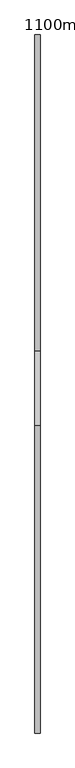
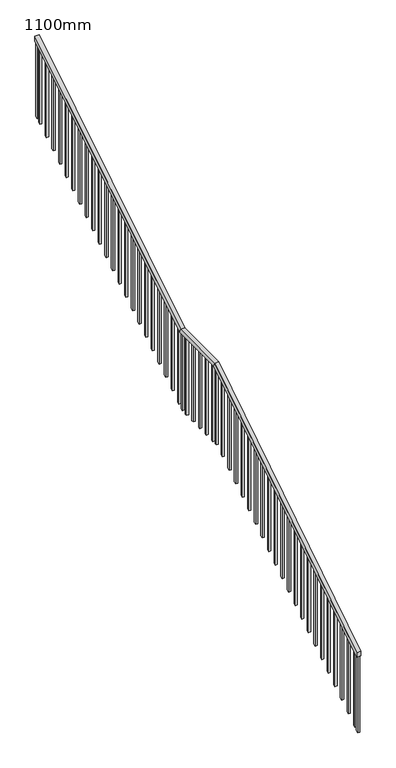
"""IFC4 building model written with IfcOpenShell, lengths in millimetres: railing geometry, 1100mm."""

from ifc_helpers import new_model, si_unit, frame, origin, place, context, project, spatial, polyline, outline, extrude, faceted_brep, source, transform, mapped, element, save


def railing_1100mm_9b3715b3(model_context):
    return source(origin(), model_context, "Body", "SolidModel", [
        faceted_brep([(-21050.0159097, -6684.456375, 1268.797954), (-21100.0159097, -6684.456375, 1268.797954), (-21100.0159097, -6684.456375, 1209.4512039), (-21050.0159097, -6684.456375, 1209.4512039), (-21050.0159097, -3684.456375, 3186.9565217), (-21100.0159097, -3684.456375, 3186.9565217), (-21100.0159097, -3669.8380579, 3136.9565217), (-21050.0159097, -3669.8380579, 3136.9565217), (-21050.0159097, -2964.456375, 3186.9565217), (-21100.0159097, -2964.456375, 3186.9565217), (-21100.0159097, -2950.192194, 3136.9565217), (-21050.0159097, -2950.192194, 3136.9565217), (-21050.0159097, 115.543625, 5100.0), (-21050.0159097, 115.543625, 5041.1402603), (-21100.0159097, 115.543625, 5041.1402603), (-21100.0159097, 115.543625, 5100.0)], [[[0, 1, 2, 3]], [[1, 0, 4, 5]], [[2, 1, 5, 6]], [[3, 2, 6, 7]], [[0, 3, 7, 4]], [[5, 4, 8, 9]], [[6, 5, 9, 10]], [[7, 6, 10, 11]], [[4, 7, 11, 8]], [[12, 13, 14, 15]], [[9, 8, 12, 15]], [[10, 9, 15, 14]], [[11, 10, 14, 13]], [[8, 11, 13, 12]]]),
        extrude(outline(polyline([(33.043625, 4009.0250545), (33.043625, 4989.8980242), (58.043625, 5005.4259745), (58.043625, 4024.5530048), (33.043625, 4009.0250545)])), frame((-21087.5159097, 0.0, 0.0), z_axis=(1.0, 0.0, 0.0), x_axis=(0.0, 1.0, 0.0)), (0.0, 0.0, 1.0), 25.0),
        extrude(outline(polyline([(-106.956375, 3922.0685328), (-106.956375, 4902.9415025), (-81.956375, 4918.4694528), (-81.956375, 3937.5964831), (-106.956375, 3922.0685328)])), frame((-21087.5159097, 0.0, 0.0), z_axis=(1.0, 0.0, 0.0), x_axis=(0.0, 1.0, 0.0)), (0.0, 0.0, 1.0), 25.0),
        extrude(outline(polyline([(-246.956375, 3835.112011), (-246.956375, 4815.9849807), (-221.956375, 4831.5129311), (-221.956375, 3850.6399613), (-246.956375, 3835.112011)])), frame((-21087.5159097, 0.0, 0.0), z_axis=(1.0, 0.0, 0.0), x_axis=(0.0, 1.0, 0.0)), (0.0, 0.0, 1.0), 25.0),
        extrude(outline(polyline([(-386.956375, 3748.1554893), (-386.956375, 4729.028459), (-361.956375, 4744.5564093), (-361.956375, 3763.6834396), (-386.956375, 3748.1554893)])), frame((-21087.5159097, 0.0, 0.0), z_axis=(1.0, 0.0, 0.0), x_axis=(0.0, 1.0, 0.0)), (0.0, 0.0, 1.0), 25.0),
        extrude(outline(polyline([(-526.956375, 3661.1989675), (-526.956375, 4642.0719373), (-501.956375, 4657.5998876), (-501.956375, 3676.7269179), (-526.956375, 3661.1989675)])), frame((-21087.5159097, 0.0, 0.0), z_axis=(1.0, 0.0, 0.0), x_axis=(0.0, 1.0, 0.0)), (0.0, 0.0, 1.0), 25.0),
        extrude(outline(polyline([(-666.956375, 3574.2424458), (-666.956375, 4555.1154155), (-641.956375, 4570.6433658), (-641.956375, 3589.7703961), (-666.956375, 3574.2424458)])), frame((-21087.5159097, 0.0, 0.0), z_axis=(1.0, 0.0, 0.0), x_axis=(0.0, 1.0, 0.0)), (0.0, 0.0, 1.0), 25.0),
        extrude(outline(polyline([(-806.956375, 3487.2859241), (-806.956375, 4468.1588938), (-781.956375, 4483.6868441), (-781.956375, 3502.8138744), (-806.956375, 3487.2859241)])), frame((-21087.5159097, 0.0, 0.0), z_axis=(1.0, 0.0, 0.0), x_axis=(0.0, 1.0, 0.0)), (0.0, 0.0, 1.0), 25.0),
        extrude(outline(polyline([(-946.956375, 3400.3294023), (-946.956375, 4381.2023721), (-921.956375, 4396.7303224), (-921.956375, 3415.8573526), (-946.956375, 3400.3294023)])), frame((-21087.5159097, 0.0, 0.0), z_axis=(1.0, 0.0, 0.0), x_axis=(0.0, 1.0, 0.0)), (0.0, 0.0, 1.0), 25.0),
        extrude(outline(polyline([(-1086.956375, 3313.3728806), (-1086.956375, 4294.2458503), (-1061.956375, 4309.7738006), (-1061.956375, 3328.9008309), (-1086.956375, 3313.3728806)])), frame((-21087.5159097, 0.0, 0.0), z_axis=(1.0, 0.0, 0.0), x_axis=(0.0, 1.0, 0.0)), (0.0, 0.0, 1.0), 25.0),
        extrude(outline(polyline([(-1226.956375, 3226.4163588), (-1226.956375, 4207.2893286), (-1201.956375, 4222.8172789), (-1201.956375, 3241.9443092), (-1226.956375, 3226.4163588)])), frame((-21087.5159097, 0.0, 0.0), z_axis=(1.0, 0.0, 0.0), x_axis=(0.0, 1.0, 0.0)), (0.0, 0.0, 1.0), 25.0),
        extrude(outline(polyline([(-1366.956375, 3139.4598371), (-1366.956375, 4120.3328068), (-1341.956375, 4135.8607571), (-1341.956375, 3154.9877874), (-1366.956375, 3139.4598371)])), frame((-21087.5159097, 0.0, 0.0), z_axis=(1.0, 0.0, 0.0), x_axis=(0.0, 1.0, 0.0)), (0.0, 0.0, 1.0), 25.0),
        extrude(outline(polyline([(-1506.956375, 3052.5033154), (-1506.956375, 4033.3762851), (-1481.956375, 4048.9042354), (-1481.956375, 3068.0312657), (-1506.956375, 3052.5033154)])), frame((-21087.5159097, 0.0, 0.0), z_axis=(1.0, 0.0, 0.0), x_axis=(0.0, 1.0, 0.0)), (0.0, 0.0, 1.0), 25.0),
        extrude(outline(polyline([(-1646.956375, 2965.5467936), (-1646.956375, 3946.4197634), (-1621.956375, 3961.9477137), (-1621.956375, 2981.0747439), (-1646.956375, 2965.5467936)])), frame((-21087.5159097, 0.0, 0.0), z_axis=(1.0, 0.0, 0.0), x_axis=(0.0, 1.0, 0.0)), (0.0, 0.0, 1.0), 25.0),
        extrude(outline(polyline([(-1786.956375, 2878.5902719), (-1786.956375, 3859.4632416), (-1761.956375, 3874.9911919), (-1761.956375, 2894.1182222), (-1786.956375, 2878.5902719)])), frame((-21087.5159097, 0.0, 0.0), z_axis=(1.0, 0.0, 0.0), x_axis=(0.0, 1.0, 0.0)), (0.0, 0.0, 1.0), 25.0),
        extrude(outline(polyline([(-1926.956375, 2791.6337502), (-1926.956375, 3772.5067199), (-1901.956375, 3788.0346702), (-1901.956375, 2807.1617005), (-1926.956375, 2791.6337502)])), frame((-21087.5159097, 0.0, 0.0), z_axis=(1.0, 0.0, 0.0), x_axis=(0.0, 1.0, 0.0)), (0.0, 0.0, 1.0), 25.0),
        extrude(outline(polyline([(-2066.956375, 2704.6772284), (-2066.956375, 3685.5501981), (-2041.956375, 3701.0781484), (-2041.956375, 2720.2051787), (-2066.956375, 2704.6772284)])), frame((-21087.5159097, 0.0, 0.0), z_axis=(1.0, 0.0, 0.0), x_axis=(0.0, 1.0, 0.0)), (0.0, 0.0, 1.0), 25.0),
        extrude(outline(polyline([(-2206.956375, 2617.7207067), (-2206.956375, 3598.5936764), (-2181.956375, 3614.1216267), (-2181.956375, 2633.248657), (-2206.956375, 2617.7207067)])), frame((-21087.5159097, 0.0, 0.0), z_axis=(1.0, 0.0, 0.0), x_axis=(0.0, 1.0, 0.0)), (0.0, 0.0, 1.0), 25.0),
        extrude(outline(polyline([(-2346.956375, 2530.7641849), (-2346.956375, 3511.6371547), (-2321.956375, 3527.165105), (-2321.956375, 2546.2921352), (-2346.956375, 2530.7641849)])), frame((-21087.5159097, 0.0, 0.0), z_axis=(1.0, 0.0, 0.0), x_axis=(0.0, 1.0, 0.0)), (0.0, 0.0, 1.0), 25.0),
        extrude(outline(polyline([(-2486.956375, 2443.8076632), (-2486.956375, 3424.6806329), (-2461.956375, 3440.2085832), (-2461.956375, 2459.3356135), (-2486.956375, 2443.8076632)])), frame((-21087.5159097, 0.0, 0.0), z_axis=(1.0, 0.0, 0.0), x_axis=(0.0, 1.0, 0.0)), (0.0, 0.0, 1.0), 25.0),
        extrude(outline(polyline([(-2626.956375, 2356.8511415), (-2626.956375, 3337.7241112), (-2601.956375, 3353.2520615), (-2601.956375, 2372.3790918), (-2626.956375, 2356.8511415)])), frame((-21087.5159097, 0.0, 0.0), z_axis=(1.0, 0.0, 0.0), x_axis=(0.0, 1.0, 0.0)), (0.0, 0.0, 1.0), 25.0),
        extrude(outline(polyline([(-2766.956375, 2269.8946197), (-2766.956375, 3250.7675894), (-2741.956375, 3266.2955398), (-2741.956375, 2285.42257), (-2766.956375, 2269.8946197)])), frame((-21087.5159097, 0.0, 0.0), z_axis=(1.0, 0.0, 0.0), x_axis=(0.0, 1.0, 0.0)), (0.0, 0.0, 1.0), 25.0),
        extrude(outline(polyline([(-2906.956375, 2182.938098), (-2906.956375, 3163.8110677), (-2881.956375, 3179.339018), (-2881.956375, 2198.4660483), (-2906.956375, 2182.938098)])), frame((-21087.5159097, 0.0, 0.0), z_axis=(1.0, 0.0, 0.0), x_axis=(0.0, 1.0, 0.0)), (0.0, 0.0, 1.0), 25.0),
        extrude(outline(polyline([(-21062.5159097, -3066.956375), (-21087.5159097, -3066.956375), (-21087.5159097, -3041.956375), (-21062.5159097, -3041.956375), (-21062.5159097, -3066.956375)])), frame((0.0, 0.0, 2133.5443962), z_axis=(0.0, 0.0, 1.0), x_axis=(1.0, 0.0, 0.0)), (0.0, 0.0, 1.0), 1003.4121256),
        extrude(outline(polyline([(-21062.5159097, -3206.956375), (-21087.5159097, -3206.956375), (-21087.5159097, -3181.956375), (-21062.5159097, -3181.956375), (-21062.5159097, -3206.956375)])), frame((0.0, 0.0, 2133.5443962), z_axis=(0.0, 0.0, 1.0), x_axis=(1.0, 0.0, 0.0)), (0.0, 0.0, 1.0), 1003.4121256),
        extrude(outline(polyline([(-21062.5159097, -3346.956375), (-21087.5159097, -3346.956375), (-21087.5159097, -3321.956375), (-21062.5159097, -3321.956375), (-21062.5159097, -3346.956375)])), frame((0.0, 0.0, 2133.5443962), z_axis=(0.0, 0.0, 1.0), x_axis=(1.0, 0.0, 0.0)), (0.0, 0.0, 1.0), 1003.4121256),
        extrude(outline(polyline([(-21062.5159097, -3486.956375), (-21087.5159097, -3486.956375), (-21087.5159097, -3461.956375), (-21062.5159097, -3461.956375), (-21062.5159097, -3486.956375)])), frame((0.0, 0.0, 2133.5443962), z_axis=(0.0, 0.0, 1.0), x_axis=(1.0, 0.0, 0.0)), (0.0, 0.0, 1.0), 1003.4121256),
        extrude(outline(polyline([(-21062.5159097, -3626.956375), (-21087.5159097, -3626.956375), (-21087.5159097, -3601.956375), (-21062.5159097, -3601.956375), (-21062.5159097, -3626.956375)])), frame((0.0, 0.0, 2133.5443962), z_axis=(0.0, 0.0, 1.0), x_axis=(1.0, 0.0, 0.0)), (0.0, 0.0, 1.0), 1003.4121256),
        extrude(outline(polyline([(-3826.956375, 2058.2984994), (-3826.956375, 3036.4972397), (-3801.956375, 3052.4818944), (-3801.956375, 2074.2831542), (-3826.956375, 2058.2984994)])), frame((-21087.5159097, 0.0, 0.0), z_axis=(1.0, 0.0, 0.0), x_axis=(0.0, 1.0, 0.0)), (0.0, 0.0, 1.0), 25.0),
        extrude(outline(polyline([(-3966.956375, 1968.7844329), (-3966.956375, 2946.9831732), (-3941.956375, 2962.9678279), (-3941.956375, 1984.7690877), (-3966.956375, 1968.7844329)])), frame((-21087.5159097, 0.0, 0.0), z_axis=(1.0, 0.0, 0.0), x_axis=(0.0, 1.0, 0.0)), (0.0, 0.0, 1.0), 25.0),
        extrude(outline(polyline([(-4106.956375, 1879.2703664), (-4106.956375, 2857.4691067), (-4081.956375, 2873.4537614), (-4081.956375, 1895.2550212), (-4106.956375, 1879.2703664)])), frame((-21087.5159097, 0.0, 0.0), z_axis=(1.0, 0.0, 0.0), x_axis=(0.0, 1.0, 0.0)), (0.0, 0.0, 1.0), 25.0),
        extrude(outline(polyline([(-4246.956375, 1789.7562999), (-4246.956375, 2767.9550402), (-4221.956375, 2783.9396949), (-4221.956375, 1805.7409547), (-4246.956375, 1789.7562999)])), frame((-21087.5159097, 0.0, 0.0), z_axis=(1.0, 0.0, 0.0), x_axis=(0.0, 1.0, 0.0)), (0.0, 0.0, 1.0), 25.0),
        extrude(outline(polyline([(-4386.956375, 1700.2422334), (-4386.956375, 2678.4409737), (-4361.956375, 2694.4256284), (-4361.956375, 1716.2268882), (-4386.956375, 1700.2422334)])), frame((-21087.5159097, 0.0, 0.0), z_axis=(1.0, 0.0, 0.0), x_axis=(0.0, 1.0, 0.0)), (0.0, 0.0, 1.0), 25.0),
        extrude(outline(polyline([(-4526.956375, 1610.7281669), (-4526.956375, 2588.9269072), (-4501.956375, 2604.9115619), (-4501.956375, 1626.7128217), (-4526.956375, 1610.7281669)])), frame((-21087.5159097, 0.0, 0.0), z_axis=(1.0, 0.0, 0.0), x_axis=(0.0, 1.0, 0.0)), (0.0, 0.0, 1.0), 25.0),
        extrude(outline(polyline([(-4666.956375, 1521.2141004), (-4666.956375, 2499.4128407), (-4641.956375, 2515.3974954), (-4641.956375, 1537.1987552), (-4666.956375, 1521.2141004)])), frame((-21087.5159097, 0.0, 0.0), z_axis=(1.0, 0.0, 0.0), x_axis=(0.0, 1.0, 0.0)), (0.0, 0.0, 1.0), 25.0),
        extrude(outline(polyline([(-4806.956375, 1431.700034), (-4806.956375, 2409.8987742), (-4781.956375, 2425.8834289), (-4781.956375, 1447.6846887), (-4806.956375, 1431.700034)])), frame((-21087.5159097, 0.0, 0.0), z_axis=(1.0, 0.0, 0.0), x_axis=(0.0, 1.0, 0.0)), (0.0, 0.0, 1.0), 25.0),
        extrude(outline(polyline([(-4946.956375, 1342.1859675), (-4946.956375, 2320.3847077), (-4921.956375, 2336.3693624), (-4921.956375, 1358.1706222), (-4946.956375, 1342.1859675)])), frame((-21087.5159097, 0.0, 0.0), z_axis=(1.0, 0.0, 0.0), x_axis=(0.0, 1.0, 0.0)), (0.0, 0.0, 1.0), 25.0),
        extrude(outline(polyline([(-5086.956375, 1252.671901), (-5086.956375, 2230.8706412), (-5061.956375, 2246.8552959), (-5061.956375, 1268.6565557), (-5086.956375, 1252.671901)])), frame((-21087.5159097, 0.0, 0.0), z_axis=(1.0, 0.0, 0.0), x_axis=(0.0, 1.0, 0.0)), (0.0, 0.0, 1.0), 25.0),
        extrude(outline(polyline([(-5226.956375, 1163.1578345), (-5226.956375, 2141.3565747), (-5201.956375, 2157.3412294), (-5201.956375, 1179.1424892), (-5226.956375, 1163.1578345)])), frame((-21087.5159097, 0.0, 0.0), z_axis=(1.0, 0.0, 0.0), x_axis=(0.0, 1.0, 0.0)), (0.0, 0.0, 1.0), 25.0),
        extrude(outline(polyline([(-5366.956375, 1073.643768), (-5366.956375, 2051.8425082), (-5341.956375, 2067.8271629), (-5341.956375, 1089.6284227), (-5366.956375, 1073.643768)])), frame((-21087.5159097, 0.0, 0.0), z_axis=(1.0, 0.0, 0.0), x_axis=(0.0, 1.0, 0.0)), (0.0, 0.0, 1.0), 25.0),
        extrude(outline(polyline([(-5506.956375, 984.1297015), (-5506.956375, 1962.3284417), (-5481.956375, 1978.3130964), (-5481.956375, 1000.1143562), (-5506.956375, 984.1297015)])), frame((-21087.5159097, 0.0, 0.0), z_axis=(1.0, 0.0, 0.0), x_axis=(0.0, 1.0, 0.0)), (0.0, 0.0, 1.0), 25.0),
        extrude(outline(polyline([(-5646.956375, 894.615635), (-5646.956375, 1872.8143752), (-5621.956375, 1888.79903), (-5621.956375, 910.6002897), (-5646.956375, 894.615635)])), frame((-21087.5159097, 0.0, 0.0), z_axis=(1.0, 0.0, 0.0), x_axis=(0.0, 1.0, 0.0)), (0.0, 0.0, 1.0), 25.0),
        extrude(outline(polyline([(-5786.956375, 805.1015685), (-5786.956375, 1783.3003087), (-5761.956375, 1799.2849635), (-5761.956375, 821.0862232), (-5786.956375, 805.1015685)])), frame((-21087.5159097, 0.0, 0.0), z_axis=(1.0, 0.0, 0.0), x_axis=(0.0, 1.0, 0.0)), (0.0, 0.0, 1.0), 25.0),
        extrude(outline(polyline([(-5926.956375, 715.587502), (-5926.956375, 1693.7862422), (-5901.956375, 1709.770897), (-5901.956375, 731.5721567), (-5926.956375, 715.587502)])), frame((-21087.5159097, 0.0, 0.0), z_axis=(1.0, 0.0, 0.0), x_axis=(0.0, 1.0, 0.0)), (0.0, 0.0, 1.0), 25.0),
        extrude(outline(polyline([(-6066.956375, 626.0734355), (-6066.956375, 1604.2721757), (-6041.956375, 1620.2568305), (-6041.956375, 642.0580902), (-6066.956375, 626.0734355)])), frame((-21087.5159097, 0.0, 0.0), z_axis=(1.0, 0.0, 0.0), x_axis=(0.0, 1.0, 0.0)), (0.0, 0.0, 1.0), 25.0),
        extrude(outline(polyline([(-6206.956375, 536.559369), (-6206.956375, 1514.7581092), (-6181.956375, 1530.742764), (-6181.956375, 552.5440237), (-6206.956375, 536.559369)])), frame((-21087.5159097, 0.0, 0.0), z_axis=(1.0, 0.0, 0.0), x_axis=(0.0, 1.0, 0.0)), (0.0, 0.0, 1.0), 25.0),
        extrude(outline(polyline([(-6346.956375, 447.0453025), (-6346.956375, 1425.2440427), (-6321.956375, 1441.2286975), (-6321.956375, 463.0299572), (-6346.956375, 447.0453025)])), frame((-21087.5159097, 0.0, 0.0), z_axis=(1.0, 0.0, 0.0), x_axis=(0.0, 1.0, 0.0)), (0.0, 0.0, 1.0), 25.0),
        extrude(outline(polyline([(-6486.956375, 357.531236), (-6486.956375, 1335.7299762), (-6461.956375, 1351.714631), (-6461.956375, 373.5158907), (-6486.956375, 357.531236)])), frame((-21087.5159097, 0.0, 0.0), z_axis=(1.0, 0.0, 0.0), x_axis=(0.0, 1.0, 0.0)), (0.0, 0.0, 1.0), 25.0),
        extrude(outline(polyline([(-6626.956375, 268.0171695), (-6626.956375, 1246.2159097), (-6601.956375, 1262.2005645), (-6601.956375, 284.0018242), (-6626.956375, 268.0171695)])), frame((-21087.5159097, 0.0, 0.0), z_axis=(1.0, 0.0, 0.0), x_axis=(0.0, 1.0, 0.0)), (0.0, 0.0, 1.0), 25.0),
        extrude(outline(polyline([(-2976.956375, 2139.4598371), (-2976.956375, 3136.9565217), (-2951.956375, 3136.9565217), (-2951.956375, 2154.9877874), (-2976.956375, 2139.4598371)])), frame((-21087.5159097, 0.0, 0.0), z_axis=(1.0, 0.0, 0.0), x_axis=(0.0, 1.0, 0.0)), (0.0, 0.0, 1.0), 25.0),
        extrude(outline(polyline([(-3696.956375, 2133.5443962), (-3696.956375, 3119.6174443), (-3671.956375, 3135.602099), (-3671.956375, 2133.5443962), (-3696.956375, 2133.5443962)])), frame((-21087.5159097, 0.0, 0.0), z_axis=(1.0, 0.0, 0.0), x_axis=(0.0, 1.0, 0.0)), (0.0, 0.0, 1.0), 25.0),
        extrude(outline(polyline([(90.543625, 4044.7393402), (90.543625, 5025.6123099), (115.543625, 5041.1402603), (115.543625, 4060.2672905), (90.543625, 4044.7393402)])), frame((-21087.5159097, 0.0, 0.0), z_axis=(1.0, 0.0, 0.0), x_axis=(0.0, 1.0, 0.0)), (0.0, 0.0, 1.0), 25.0),
        extrude(outline(polyline([(-6684.456375, 231.2524636), (-6684.456375, 1209.4512039), (-6659.456375, 1225.4358586), (-6659.456375, 247.2371184), (-6684.456375, 231.2524636)])), frame((-21087.5159097, 0.0, 0.0), z_axis=(1.0, 0.0, 0.0), x_axis=(0.0, 1.0, 0.0)), (0.0, 0.0, 1.0), 25.0),
    ])


if __name__ == "__main__":
    model = new_model("IFC4")
    model_context = context("Model", 3, world=origin())
    ifc_project = project(units=[si_unit("LENGTHUNIT", "METRE", prefix="MILLI")], contexts=[model_context])
    site = spatial("IfcSite", under=ifc_project)
    building = spatial("IfcBuilding", under=site)
    placement = place(None, origin())
    railing_1100mm_shape = railing_1100mm_9b3715b3(model_context)
    element("IfcRailing", 1, ObjectType="1100mm", at=placement, inside=building, context=model_context, shape_type="MappedRepresentation", body=[
        mapped(railing_1100mm_shape, transform((0.0, 0.0, 0.0), x_axis=(1.0, 0.0, 0.0), y_axis=(0.0, 1.0, 0.0), z_axis=(0.0, 0.0, 1.0))),
    ])
    save(model, "model.ifc")
